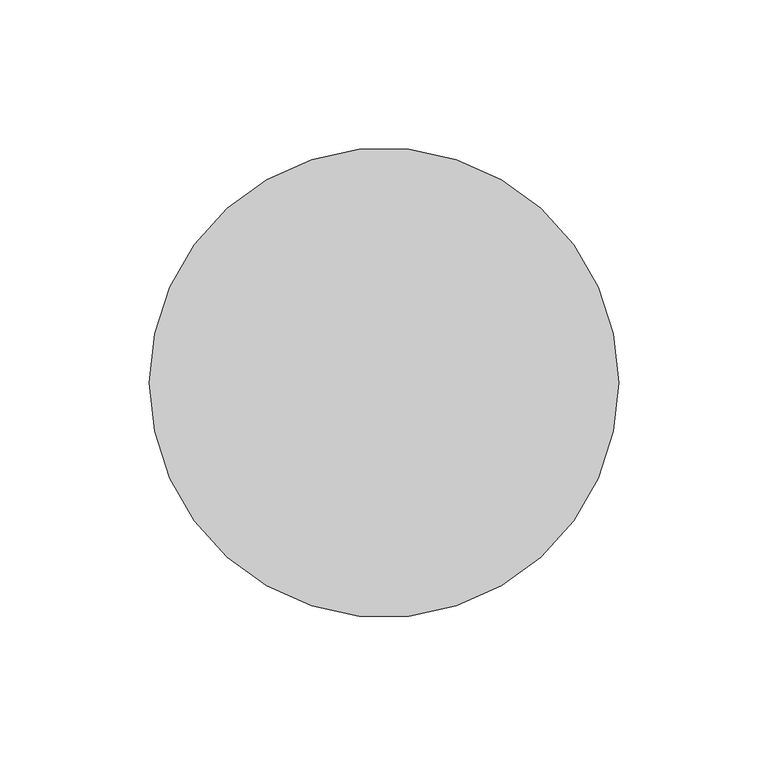
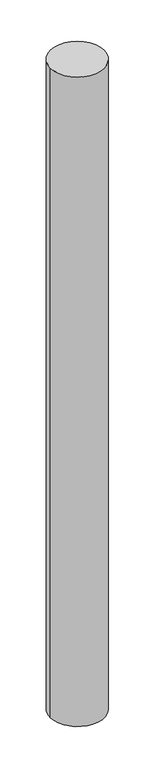
"""IFC4 building model written with IfcOpenShell, lengths in millimetres: proxy geometry, NLRS_71_GM_WPB_afschermpaal aardebaan_gen_rsf : afschermpaal aardebaan dxl 159x2000mm."""

from ifc_helpers import new_model, si_unit, point, frame, frame_2d, origin, place, context, project, spatial, circle_curve, trimmed, segment, composite_curve, outline, extrude, source, transform, mapped, element, save


def generic_models_f4b89450(model_context):
    return source(origin(), model_context, "Body", "SweptSolid", [
        extrude(outline(composite_curve([segment(trimmed(circle_curve(frame_2d((1.2, -75.0)), 78.5), [point((-77.3, -75.0))], [point((79.7, -75.0))], False, "CARTESIAN"), True, "CONTINUOUS"), segment(trimmed(circle_curve(frame_2d((1.2, -75.0)), 78.5), [point((79.7, -75.0))], [point((-77.3, -75.0))], False, "CARTESIAN"), True, "CONTINUOUS")], self_intersect=False)), frame((0.0, 0.0, -1000.0), z_axis=(0.0, 0.0, 1.0), x_axis=(1.0, 0.0, 0.0)), (0.0, 0.0, 1.0), 2000.0),
    ])


if __name__ == "__main__":
    model = new_model("IFC4")
    model_context = context("Model", 3, world=origin())
    ifc_project = project(units=[si_unit("LENGTHUNIT", "METRE", prefix="MILLI")], contexts=[model_context])
    site = spatial("IfcSite", under=ifc_project)
    building = spatial("IfcBuilding", under=site)
    placement = place(None, origin())
    generic_models_shape = generic_models_f4b89450(model_context)
    element("IfcBuildingElementProxy", 1, Name="NLRS_71_GM_WPB_afschermpaal aardebaan_gen_rsf : afschermpaal aardebaan dxl 159x2000mm", ObjectType="NLRS_71_GM_WPB_afschermpaal aardebaan_gen_rsf : afschermpaal aardebaan dxl 159x2000mm", at=placement, inside=building, context=model_context, shape_type="MappedRepresentation", body=[
        mapped(generic_models_shape, transform((0.0, 0.0, 0.0), x_axis=(1.0, 0.0, 0.0), y_axis=(0.0, 1.0, 0.0), z_axis=(0.0, 0.0, 1.0))),
    ])
    save(model, "model.ifc")

# Revit data of these elements
# Type "NLRS_71_GM_WPB_afschermpaal aardebaan_gen_rsf : afschermpaal aardebaan dxl 159x2000mm"
#   Type IFC Predefined Type = "USERDEFINED"
#   Export Type to IFC As = "IfcGeographicElementType"
#   Type IfcGUID = "05J6pyYiTDtR2exmlhyPlb"
#   IfcName[Type] = "afschermpaal aardebaan dxl 159x2000mm"
#   IfcDescription[Type] = "verkeerspaal dxl 159x2000mm"
#   IfcObjectType[Type] = "BOLLARD"
#   IfcExportAs[Type] = "IfcGeographicElementType"
#   IfcExportType[Type] = "USERDEFINED"
#   NLRS_C_revit_versie = "2021"
#   NLRS_C_materiaal_afwerking [instance default] = ""
#   NLRS_C_content_versie = ""
#   NLRS_C_content_provider = ""
#   NLRS_C_content_handleiding = ""
#   NLRS_C_content_datum_uitgifte = ""
#   NLRS_C_content_datum_gewijzigd = ""
#   NLRS_C_content_creator = ""
#   NLRS_C_brandwerendheid_text [instance default] = ""
#   NLRS_C_brandwerendheid_EI_text [instance default] = ""
#   Model = "generiek"
#   Manufacturer = "generiek"
#   Description = "verkeerspaal dxl 159x2000mm"
#   Assembly Code = "71.10"
#   NLRS_S_gewicht [instance default] = 0.00 kg
#   NLRS_C_radius = 78.50 mm
#   NLRS_C_offset [instance default] = 0.00 mm
#   NLRS_C_hoogte = 2000.00 mm
#   NLRS_C_diepte = 1000.00 mm
#   NLRS_C_buiten [instance default] = yes
#   NLRS_C_brandwerend [instance default] = yes
#   NLRS_C_brandbaar [instance default] = yes
#   NLRS_C_materiaal = none
#   URL = ""
#   Default Elevation = 0
